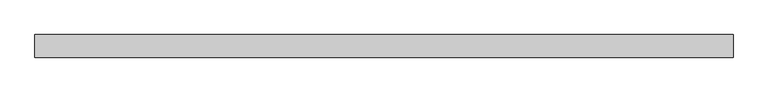
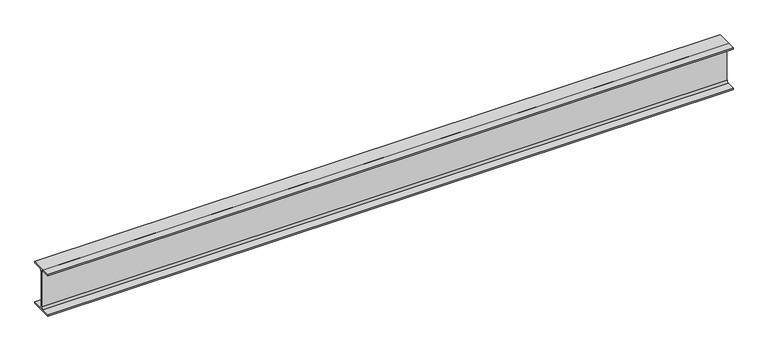
"""IFC4 building model written with IfcOpenShell, lengths in millimetres: beam geometry, 0912_Steel Framing_H-KSD3502 : H_SB_ASB_H-250x125x6x9."""

from ifc_helpers import new_model, si_unit, point, frame, frame_2d, origin, place, context, project, spatial, polyline, circle_curve, trimmed, segment, composite_curve, outline, extrude, source, transform, mapped, element, save


def beam_97186c57(model_context):
    return source(origin(), model_context, "Body", "SweptSolid", [
        extrude(outline(composite_curve([segment(polyline([(62.5, -116.0), (62.5, -125.0), (-62.5, -125.0), (-62.5, -116.0), (-15.0, -116.0)]), True, "CONTINUOUS"), segment(trimmed(circle_curve(frame_2d((-15.0, -104.0)), 12.0), [point((-15.0, -116.0))], [point((-3.0, -104.0))], True, "CARTESIAN"), True, "CONTINUOUS"), segment(polyline([(-3.0, -104.0), (-3.0, 104.0)]), True, "CONTINUOUS"), segment(trimmed(circle_curve(frame_2d((-15.0, 104.0)), 12.0), [point((-3.0, 104.0))], [point((-15.0, 116.0))], True, "CARTESIAN"), True, "CONTINUOUS"), segment(polyline([(-15.0, 116.0), (-62.5, 116.0), (-62.5, 125.0), (62.5, 125.0), (62.5, 116.0), (15.0, 116.0)]), True, "CONTINUOUS"), segment(trimmed(circle_curve(frame_2d((15.0, 104.0)), 12.0), [point((15.0, 116.0))], [point((3.0, 104.0))], True, "CARTESIAN"), True, "CONTINUOUS"), segment(polyline([(3.0, 104.0), (3.0, -104.0)]), True, "CONTINUOUS"), segment(trimmed(circle_curve(frame_2d((15.0, -104.0)), 12.0), [point((3.0, -104.0))], [point((15.0, -116.0))], True, "CARTESIAN"), True, "CONTINUOUS"), segment(polyline([(15.0, -116.0), (62.5, -116.0)]), True, "CONTINUOUS")], self_intersect=False)), frame((-1830.0829189, 0.0, 0.0), z_axis=(1.0, 0.0, 0.0), x_axis=(0.0, 1.0, 0.0)), (0.0, 0.0, 1.0), 3859.8829189),
    ])


if __name__ == "__main__":
    model = new_model("IFC4")
    model_context = context("Model", 3, world=origin())
    ifc_project = project(units=[si_unit("LENGTHUNIT", "METRE", prefix="MILLI")], contexts=[model_context])
    site = spatial("IfcSite", under=ifc_project)
    building = spatial("IfcBuilding", under=site)
    placement = place(None, origin())
    beam_shape = beam_97186c57(model_context)
    element("IfcBeam", 1, ObjectType="0912_Steel Framing_H-KSD3502 : H_SB_ASB_H-250x125x6x9", at=placement, inside=building, context=model_context, shape_type="MappedRepresentation", body=[
        mapped(beam_shape, transform((0.0, 0.0, 0.0), x_axis=(1.0, 0.0, 0.0), y_axis=(0.0, 1.0, 0.0), z_axis=(0.0, 0.0, 1.0))),
    ])
    save(model, "model.ifc")

# Revit data of these elements
# Type "0912_Steel Framing_H-KSD3502 : H_SB_ASB_H-250x125x6x9"
#   H_WM Code_1 = "S01AA003-00001 | Main Steel Structure Fabrication Work | Shelter/Building | Light Steel - Standard (30KG/M>Weight) | Material: (   )"
#   H_WM Code_2 = "S03AA029-00001 | Main Steel Structure Erection Work | Shelter/Building | Light Steel (30KG/M>Weight) | Material: (   )"
#   H_WM Code_3 = "S01AA010-00001 | Main Steel Structure Fabrication Work | Shelter/Building | Steel Painting/Coating | for Non-Fireproofed Steel Surface, Surface Preparation, Primer, Second & Final Coat | Material: (   )"
#   H_Q'ty Cal Type Tag = "SB-Q2"
#   Width = 12.5 cm
#   Web Thickness = 0.6 cm
#   Web Fillet = 1.2 cm
#   Warping Constant = 42539.8 cm⁶
#   W = 0
#   Torsional Moment of Inertia = 7.8102 cm⁴
#   Section Area = 37.66 cm²
#   Plastic Modulus weak axis = 73.1 cm³
#   Plastic Modulus strong axis = 366.0 cm³
#   Perimeter = 0.97 m²/m
#   Nominal Weight = 29.60 kgf/m
#   Moment of Inertia weak axis = 294.00 cm⁴
#   Moment of Inertia strong axis = 4050.00 cm⁴
#   Height = 25.0 cm
#   Flange Thickness = 0.9 cm
#   Elastic Modulus weak axis = 47.0 cm³
#   Elastic Modulus strong axis = 324.0 cm³
#   Centroid Vertical = 12.5 cm
#   Centroid Horizontal = 6.25 cm
#   Ix = 40500000
#   Length [instance default] = 1.5240 m
#   Zx = 366000
#   b = 0.1250 m
#   h = 0.2500 m
#   r = 0.0120 m
#   s = 0.0060 m
#   t = 0.0090 m
#   A = 0.003766 m²
#   Structural Material [instance default] = Steel, 45-345
#   Assembly Code = ""
# Element 1 (IfcBeam, "0912_Steel Framing_H-KSD3502 : H_SB_ASB_H-250x125x6x9")
#   Structural Material = none
# Materials
#   "Steel, 45-345": class "Metal", colour RGB 189 187 185, transparency 0, Description = "Steel 345 MPa", Cost = 0
